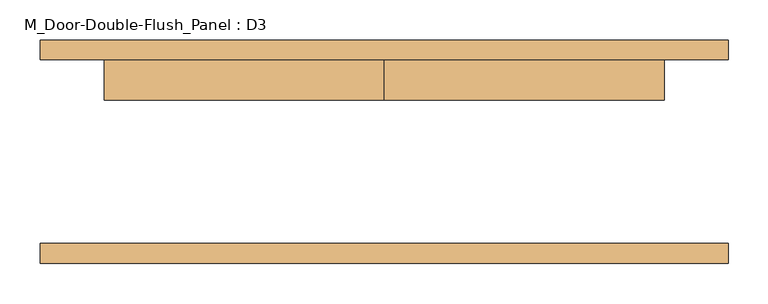
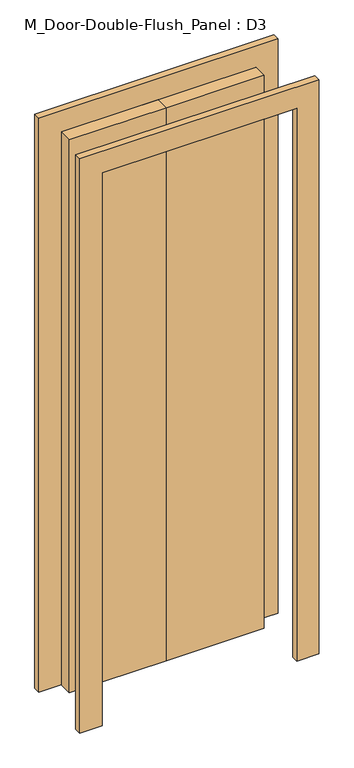
"""IFC4 building model written with IfcOpenShell, lengths in millimetres: door geometry, M_Door-Double-Flush_Panel : D3."""

from ifc_helpers import new_model, si_unit, frame, origin, origin_with_axes, place, context, project, spatial, polyline, outline, extrude, source, transform, mapped, element, save


def m_door_double_flush_panel_d3_ec03c414(model_context):
    return source(origin(), model_context, "Body", "SweptSolid", [
        extrude(outline(polyline([(2100.0, -350.0), (2100.0, 350.0), (0.0, 350.0), (0.0, 430.0), (2180.0, 430.0), (2180.0, -430.0), (0.0, -430.0), (0.0, -350.0), (2100.0, -350.0)])), frame((0.0, -140.0, 0.0), z_axis=(0.0, 1.0, 0.0), x_axis=(0.0, 0.0, 1.0)), (0.0, 0.0, 1.0), 25.0),
        extrude(outline(polyline([(2100.0, -350.0), (2100.0, 350.0), (0.0, 350.0), (0.0, 430.0), (2180.0, 430.0), (2180.0, -430.0), (0.0, -430.0), (0.0, -350.0), (2100.0, -350.0)])), frame((0.0, 115.0, 0.0), z_axis=(0.0, 1.0, 0.0), x_axis=(0.0, 0.0, 1.0)), (0.0, 0.0, 1.0), 25.0),
        extrude(outline(polyline([(0.0, 115.0), (350.0, 115.0), (350.0, 65.0), (0.0, 65.0), (0.0, 115.0)])), origin_with_axes(), (0.0, 0.0, 1.0), 2100.0),
        extrude(outline(polyline([(-350.0, 115.0), (0.0, 115.0), (0.0, 65.0), (-350.0, 65.0), (-350.0, 115.0)])), origin_with_axes(), (0.0, 0.0, 1.0), 2100.0),
    ])


if __name__ == "__main__":
    model = new_model("IFC4")
    model_context = context("Model", 3, world=origin())
    ifc_project = project(units=[si_unit("LENGTHUNIT", "METRE", prefix="MILLI")], contexts=[model_context])
    site = spatial("IfcSite", under=ifc_project)
    building = spatial("IfcBuilding", under=site)
    placement = place(None, origin())
    m_door_double_flush_panel_d3_shape = m_door_double_flush_panel_d3_ec03c414(model_context)
    element("IfcDoor", 1, ObjectType="M_Door-Double-Flush_Panel : D3", at=placement, inside=building, context=model_context, shape_type="MappedRepresentation", body=[
        mapped(m_door_double_flush_panel_d3_shape, transform((0.0, 0.0, 0.0), x_axis=(1.0, 0.0, 0.0), y_axis=(0.0, 1.0, 0.0), z_axis=(0.0, 0.0, 1.0))),
    ])
    save(model, "model.ifc")

# Revit data of these elements
# Type "M_Door-Double-Flush_Panel : D3"
#   Type Mark = "57"
#   Construction Type Id = "DOOR"
#   Assembly Code = "C1020"
#   Analytic Construction = "Wooden"
#   Thickness = 5 cm
#   Thermal Resistance (R) = 0.455703 (m²·K)/W
#   Swing Angle [instance default] = 90.00°
#   Panel Width = 35 cm
#   Heat Transfer Coefficient (U) = 2.19465 W/(m²·K)
#   Height = 210 cm
#   Trim Projection Ext = 2.5 cm
#   Trim Projection Int = 2.5 cm
#   Trim Width = 8 cm
#   Width = 70 cm
#   Panel Material = Wood - Birch - Solid Stained Light Low Gloss
#   Trim Material = Paint - Sienna
#   Visual Light Transmittance = 0
#   Solar Heat Gain Coefficient = 0
#   Function = (empty or 0)
#   Wall Closure = (empty or 0)
# Element 1 (IfcDoor, "M_Door-Double-Flush_Panel : D3")
#   Materials on its faces: "Paint - Sienna", "Wood - Birch - Solid Stained Light Low Gloss"
# Materials
#   "Wood - Birch - Solid Stained Light Low Gloss": class "Wood", colour RGB 210 159 95, transparency 0, Cost = 0
#   "Paint - Sienna": class "Miscellaneous", colour RGB 118 70 51, transparency 0, Cost = 0
